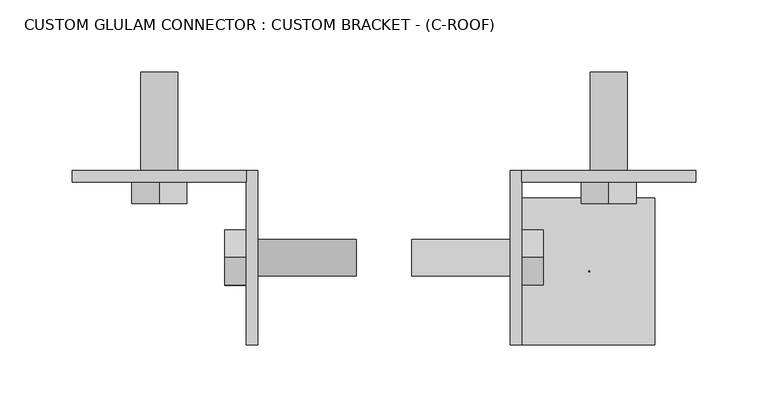
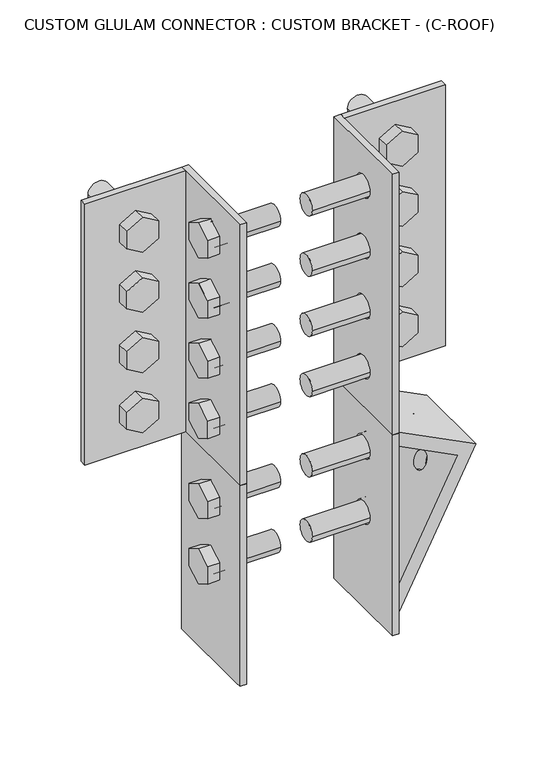
"""IFC4 building model written with IfcOpenShell, lengths in millimetres: fastener geometry, CUSTOM GLULAM CONNECTOR : CUSTOM BRACKET - (C-ROOF)."""

from ifc_helpers import new_model, si_unit, point, frame, frame_2d, origin, place, context, project, spatial, polyline, circle_curve, trimmed, segment, composite_curve, outline, extrude, source, transform, mapped, element, save
from ifc_brep_helpers import plane_surface, revolved_surface, advanced_brep


def custom_glulam_connector_custom_bracket_c_roof_f3df198d(model_context):
    return source(origin(), model_context, "Body", "SolidModel", [
        advanced_brep(
        [(-95.25, 60.325, 7.9375), (-95.25, 60.325, 261.9375), (-87.3125, 60.325, 261.9375), (-87.3125, 60.325, 7.9375), (-95.25, -60.325, 261.9375), (-95.25, -60.325, 7.9375), (-87.3125, -60.325, 7.9375), (-87.3125, -60.325, 261.9375), (-95.25, 13.890625, 128.5875), (-87.3125, 13.890625, 128.5875), (-87.3125, -13.890625, 128.5875), (-95.25, -13.890625, 128.5875), (-95.25, -52.3875, 261.9375), (-95.25, -52.3875, 7.9375), (-95.25, -13.890625, 211.1375), (-95.25, 13.890625, 211.1375), (-87.3125, 13.890625, 211.1375), (-87.3125, -13.890625, 211.1375)],
        [
            (0, 1),
            (1, 2),
            (2, 3),
            (3, 0),
            (4, 5),
            (5, 6),
            (6, 7),
            (7, 4),
            (8, 9),
            (9, 10, circle_curve(frame((-87.3125, 0.0, 128.5875), z_axis=(1.0, 0.0, 0.0), x_axis=(0.0, -1.0, 0.0)), 13.890625)),
            (10, 11),
            (11, 8, circle_curve(frame((-95.25, 0.0, 128.5875), z_axis=(-1.0, 0.0, 0.0), x_axis=(0.0, -1.0, 0.0)), 13.890625)),
            (4, 12),
            (12, 1),
            (0, 13),
            (13, 5),
            (11, 8, circle_curve(frame((-95.25, 0.0, 128.5875), z_axis=(1.0, 0.0, 0.0), x_axis=(0.0, -1.0, 0.0)), 13.890625)),
            (14, 15, circle_curve(frame((-95.25, 0.0, 211.1375), z_axis=(1.0, 0.0, 0.0), x_axis=(0.0, -1.0, 0.0)), 13.890625)),
            (15, 14, circle_curve(frame((-95.25, 0.0, 211.1375), z_axis=(1.0, 0.0, 0.0), x_axis=(0.0, -1.0, 0.0)), 13.890625)),
            (16, 15),
            (14, 17),
            (17, 16, circle_curve(frame((-87.3125, 0.0, 211.1375), z_axis=(1.0, 0.0, 0.0), x_axis=(0.0, -1.0, 0.0)), 13.890625)),
            (16, 17, circle_curve(frame((-87.3125, 0.0, 211.1375), z_axis=(1.0, 0.0, 0.0), x_axis=(0.0, -1.0, 0.0)), 13.890625)),
            (10, 9, circle_curve(frame((-87.3125, 0.0, 128.5875), z_axis=(1.0, 0.0, 0.0), x_axis=(0.0, -1.0, 0.0)), 13.890625)),
            (6, 3),
            (2, 7),
        ],
        [
            plane_surface(frame((-95.25, 60.325, 261.9375), z_axis=(0.0, 1.0, 0.0), x_axis=(1.0, 0.0, 0.0))),
            plane_surface(frame((-95.25, -60.325, 7.9375), z_axis=(0.0, -1.0, 0.0), x_axis=(1.0, 0.0, 0.0))),
            revolved_surface(polyline([(-95.25, -13.890625, 128.5875), (-87.3125, -13.890625, 128.5875)]), (-87.3125, 0.0, 128.5875), (-1.0, 0.0, 0.0)),
            plane_surface(frame((-95.25, 60.325, 261.9375), z_axis=(-1.0, 0.0, 0.0), x_axis=(0.0, 1.0, 0.0))),
            revolved_surface(polyline([(-95.25, -13.890625, 211.1375), (-87.3125, -13.890625, 211.1375)]), (-87.3125, 0.0, 211.1375), (-1.0, 0.0, 0.0)),
            plane_surface(frame((-87.3125, 60.325, 261.9375), z_axis=(1.0, 0.0, 0.0), x_axis=(0.0, -1.0, 0.0))),
            plane_surface(frame((-95.25, -60.325, 261.9375), z_axis=(0.0, 0.0, 1.0), x_axis=(1.0, 0.0, 0.0))),
            plane_surface(frame((-95.25, 60.325, 7.9375), z_axis=(0.0, 0.0, -1.0), x_axis=(1.0, 0.0, 0.0))),
        ],
        [
            (0, [[1, 2, 3, 4]]),
            (1, [[5, 6, 7, 8]]),
            (2, [[9, 10, 11, 12]]),
            (3, [[13, 14, -1, 15, 16, -5], [17, -12], [18, 19]]),
            (4, [[20, -18, 21, 22]]),
            (4, [[-20, 23, -21, -19]]),
            (2, [[-9, -17, -11, 24]]),
            (5, [[-7, 25, -3, 26], [-22, -23], [-24, -10]]),
            (6, [[-14, -13, -8, -26, -2]]),
            (7, [[-16, -15, -4, -25, -6]]),
        ],
    ),
        extrude(outline(polyline([(19.05, 222.1360226), (19.05, 200.1389774), (0.0, 189.1404547), (-19.05, 200.1389774), (-19.05, 222.1360226), (0.0, 233.1345453), (19.05, 222.1360226)])), frame((-110.2320312, 0.0, 0.0), z_axis=(1.0, 0.0, 0.0), x_axis=(0.0, 1.0, 0.0)), (0.0, 0.0, 1.0), 14.9820312),
        extrude(outline(composite_curve([segment(trimmed(circle_curve(frame_2d((0.0, 211.1375)), 12.7), [point((12.7, 211.1375))], [point((-12.7, 211.1375))], False, "CARTESIAN"), True, "CONTINUOUS"), segment(trimmed(circle_curve(frame_2d((0.0, 211.1375)), 12.7), [point((-12.7, 211.1375))], [point((12.7, 211.1375))], False, "CARTESIAN"), True, "CONTINUOUS")], self_intersect=False)), frame((-95.25, 0.0, 0.0), z_axis=(1.0, 0.0, 0.0), x_axis=(0.0, 1.0, 0.0)), (0.0, 0.0, 1.0), 76.2),
        extrude(outline(polyline([(19.05, 139.5860226), (19.05, 117.5889774), (0.0, 106.5904547), (-19.05, 117.5889774), (-19.05, 139.5860226), (0.0, 150.5845453), (19.05, 139.5860226)])), frame((-110.2320312, 0.0, 0.0), z_axis=(1.0, 0.0, 0.0), x_axis=(0.0, 1.0, 0.0)), (0.0, 0.0, 1.0), 14.9820312),
        extrude(outline(composite_curve([segment(trimmed(circle_curve(frame_2d((0.0, 128.5875)), 12.7), [point((12.7, 128.5875))], [point((-12.7, 128.5875))], False, "CARTESIAN"), True, "CONTINUOUS"), segment(trimmed(circle_curve(frame_2d((0.0, 128.5875)), 12.7), [point((-12.7, 128.5875))], [point((12.7, 128.5875))], False, "CARTESIAN"), True, "CONTINUOUS")], self_intersect=False)), frame((-95.25, 0.0, 0.0), z_axis=(1.0, 0.0, 0.0), x_axis=(0.0, 1.0, 0.0)), (0.0, 0.0, 1.0), 76.2),
        extrude(outline(polyline([(19.05, 222.1360226), (19.05, 200.1389774), (0.0, 189.1404547), (-19.05, 200.1389774), (-19.05, 222.1360226), (0.0, 233.1345453), (19.05, 222.1360226)])), frame((-110.2320312, 0.0, 0.0), z_axis=(1.0, 0.0, 0.0), x_axis=(0.0, 1.0, 0.0)), (0.0, 0.0, 1.0), 14.9820312),
        extrude(outline(composite_curve([segment(trimmed(circle_curve(frame_2d((0.0, 211.1375)), 12.7), [point((12.7, 211.1375))], [point((-12.7, 211.1375))], False, "CARTESIAN"), True, "CONTINUOUS"), segment(trimmed(circle_curve(frame_2d((0.0, 211.1375)), 12.7), [point((-12.7, 211.1375))], [point((12.7, 211.1375))], False, "CARTESIAN"), True, "CONTINUOUS")], self_intersect=False)), frame((-95.25, 0.0, 0.0), z_axis=(1.0, 0.0, 0.0), x_axis=(0.0, 1.0, 0.0)), (0.0, 0.0, 1.0), 76.2),
        advanced_brep(
        [(95.25, 60.325, 7.9375), (87.3125, 60.325, 7.9375), (87.3125, 60.325, 261.9375), (95.25, 60.325, 261.9375), (95.25, -60.325, 261.9375), (87.3125, -60.325, 261.9375), (87.3125, -60.325, 7.9375), (95.25, -60.325, 7.9375), (95.25, 13.890625, 128.5875), (95.25, -13.890625, 128.5875), (87.3125, -13.890625, 128.5875), (87.3125, 13.890625, 128.5875), (95.25, -52.3875, 7.9375), (95.25, -52.3875, 261.9375), (95.25, -13.890625, 211.1375), (95.25, 13.890625, 211.1375), (87.3125, 13.890625, 211.1375), (87.3125, -13.890625, 211.1375)],
        [
            (0, 1),
            (1, 2),
            (2, 3),
            (3, 0),
            (4, 5),
            (5, 6),
            (6, 7),
            (7, 4),
            (8, 9, circle_curve(frame((95.25, 0.0, 128.5875), z_axis=(1.0, 0.0, 0.0), x_axis=(0.0, -1.0, 0.0)), 13.890625)),
            (9, 10),
            (10, 11, circle_curve(frame((87.3125, 0.0, 128.5875), z_axis=(-1.0, 0.0, 0.0), x_axis=(0.0, -1.0, 0.0)), 13.890625)),
            (11, 8),
            (7, 12),
            (12, 0),
            (3, 13),
            (13, 4),
            (14, 15, circle_curve(frame((95.25, 0.0, 211.1375), z_axis=(-1.0, 0.0, 0.0), x_axis=(0.0, -1.0, 0.0)), 13.890625)),
            (15, 14, circle_curve(frame((95.25, 0.0, 211.1375), z_axis=(-1.0, 0.0, 0.0), x_axis=(0.0, -1.0, 0.0)), 13.890625)),
            (8, 9, circle_curve(frame((95.25, 0.0, 128.5875), z_axis=(-1.0, 0.0, 0.0), x_axis=(0.0, -1.0, 0.0)), 13.890625)),
            (16, 17, circle_curve(frame((87.3125, 0.0, 211.1375), z_axis=(-1.0, 0.0, 0.0), x_axis=(0.0, -1.0, 0.0)), 13.890625)),
            (17, 14),
            (15, 16),
            (17, 16, circle_curve(frame((87.3125, 0.0, 211.1375), z_axis=(-1.0, 0.0, 0.0), x_axis=(0.0, -1.0, 0.0)), 13.890625)),
            (11, 10, circle_curve(frame((87.3125, 0.0, 128.5875), z_axis=(-1.0, 0.0, 0.0), x_axis=(0.0, -1.0, 0.0)), 13.890625)),
            (5, 2),
            (1, 6),
        ],
        [
            plane_surface(frame((95.25, 60.325, 261.9375), z_axis=(0.0, 1.0, 0.0), x_axis=(-1.0, 0.0, 0.0))),
            plane_surface(frame((95.25, -60.325, 7.9375), z_axis=(0.0, -1.0, 0.0), x_axis=(-1.0, 0.0, 0.0))),
            revolved_surface(polyline([(95.25, -13.890625, 128.5875), (87.3125, -13.890625, 128.5875)]), (87.3125, 0.0, 128.5875), (1.0, 0.0, 0.0)),
            plane_surface(frame((95.25, 60.325, 261.9375), z_axis=(1.0, 0.0, 0.0), x_axis=(0.0, 1.0, 0.0))),
            revolved_surface(polyline([(95.25, -13.890625, 211.1375), (87.3125, -13.890625, 211.1375)]), (87.3125, 0.0, 211.1375), (1.0, 0.0, 0.0)),
            plane_surface(frame((87.3125, 60.325, 261.9375), z_axis=(-1.0, 0.0, 0.0), x_axis=(0.0, -1.0, 0.0))),
            plane_surface(frame((95.25, -60.325, 261.9375), z_axis=(0.0, 0.0, 1.0), x_axis=(-1.0, 0.0, 0.0))),
            plane_surface(frame((95.25, 60.325, 7.9375), z_axis=(0.0, 0.0, -1.0), x_axis=(-1.0, 0.0, 0.0))),
        ],
        [
            (0, [[1, 2, 3, 4]]),
            (1, [[5, 6, 7, 8]]),
            (2, [[9, 10, 11, 12]]),
            (3, [[-8, 13, 14, -4, 15, 16], [17, 18], [-9, 19]]),
            (4, [[20, 21, -18, 22]]),
            (4, [[-17, -21, 23, -22]]),
            (2, [[24, -10, -19, -12]]),
            (5, [[25, -2, 26, -6], [-23, -20], [-11, -24]]),
            (6, [[-3, -25, -5, -16, -15]]),
            (7, [[-7, -26, -1, -14, -13]]),
        ],
    ),
        extrude(outline(polyline([(19.05, 222.1360226), (19.05, 200.1389774), (0.0, 189.1404547), (-19.05, 200.1389774), (-19.05, 222.1360226), (0.0, 233.1345453), (19.05, 222.1360226)])), frame((95.25, 0.0, 0.0), z_axis=(1.0, 0.0, 0.0), x_axis=(0.0, 1.0, 0.0)), (0.0, 0.0, 1.0), 14.9820312),
        extrude(outline(composite_curve([segment(trimmed(circle_curve(frame_2d((0.0, 211.1375)), 12.7), [point((12.7, 211.1375))], [point((-12.7, 211.1375))], False, "CARTESIAN"), True, "CONTINUOUS"), segment(trimmed(circle_curve(frame_2d((0.0, 211.1375)), 12.7), [point((-12.7, 211.1375))], [point((12.7, 211.1375))], False, "CARTESIAN"), True, "CONTINUOUS")], self_intersect=False)), frame((19.05, 0.0, 0.0), z_axis=(1.0, 0.0, 0.0), x_axis=(0.0, 1.0, 0.0)), (0.0, 0.0, 1.0), 76.2),
        extrude(outline(polyline([(19.05, 139.5860226), (19.05, 117.5889774), (0.0, 106.5904547), (-19.05, 117.5889774), (-19.05, 139.5860226), (0.0, 150.5845453), (19.05, 139.5860226)])), frame((95.25, 0.0, 0.0), z_axis=(1.0, 0.0, 0.0), x_axis=(0.0, 1.0, 0.0)), (0.0, 0.0, 1.0), 14.9820312),
        extrude(outline(composite_curve([segment(trimmed(circle_curve(frame_2d((0.0, 128.5875)), 12.7), [point((12.7, 128.5875))], [point((-12.7, 128.5875))], False, "CARTESIAN"), True, "CONTINUOUS"), segment(trimmed(circle_curve(frame_2d((0.0, 128.5875)), 12.7), [point((-12.7, 128.5875))], [point((12.7, 128.5875))], False, "CARTESIAN"), True, "CONTINUOUS")], self_intersect=False)), frame((19.05, 0.0, 0.0), z_axis=(1.0, 0.0, 0.0), x_axis=(0.0, 1.0, 0.0)), (0.0, 0.0, 1.0), 76.2),
        extrude(outline(polyline([(19.05, 222.1360226), (19.05, 200.1389774), (0.0, 189.1404547), (-19.05, 200.1389774), (-19.05, 222.1360226), (0.0, 233.1345453), (19.05, 222.1360226)])), frame((95.25, 0.0, 0.0), z_axis=(1.0, 0.0, 0.0), x_axis=(0.0, 1.0, 0.0)), (0.0, 0.0, 1.0), 14.9820312),
        extrude(outline(composite_curve([segment(trimmed(circle_curve(frame_2d((0.0, 211.1375)), 12.7), [point((12.7, 211.1375))], [point((-12.7, 211.1375))], False, "CARTESIAN"), True, "CONTINUOUS"), segment(trimmed(circle_curve(frame_2d((0.0, 211.1375)), 12.7), [point((-12.7, 211.1375))], [point((12.7, 211.1375))], False, "CARTESIAN"), True, "CONTINUOUS")], self_intersect=False)), frame((19.05, 0.0, 0.0), z_axis=(1.0, 0.0, 0.0), x_axis=(0.0, 1.0, 0.0)), (0.0, 0.0, 1.0), 76.2),
        extrude(outline(polyline([(592.1375, -215.9), (261.9375, -215.9), (261.9375, -95.25), (592.1375, -95.25), (592.1375, -215.9)]), holes=[composite_curve([segment(trimmed(circle_curve(frame_2d((465.1375, -155.575)), 13.890625), [point((465.1375, -169.465625))], [point((465.1375, -141.684375))], True, "CARTESIAN"), True, "CONTINUOUS"), segment(trimmed(circle_curve(frame_2d((465.1375, -155.575)), 13.890625), [point((465.1375, -141.684375))], [point((465.1375, -169.465625))], True, "CARTESIAN"), True, "CONTINUOUS")], self_intersect=False), composite_curve([segment(trimmed(circle_curve(frame_2d((388.9375, -155.575)), 13.890625), [point((388.9375, -169.465625))], [point((388.9375, -141.684375))], True, "CARTESIAN"), True, "CONTINUOUS"), segment(trimmed(circle_curve(frame_2d((388.9375, -155.575)), 13.890625), [point((388.9375, -141.684375))], [point((388.9375, -169.465625))], True, "CARTESIAN"), True, "CONTINUOUS")], self_intersect=False), composite_curve([segment(trimmed(circle_curve(frame_2d((312.7375, -155.575)), 13.890625), [point((312.7375, -169.465625))], [point((312.7375, -141.684375))], True, "CARTESIAN"), True, "CONTINUOUS"), segment(trimmed(circle_curve(frame_2d((312.7375, -155.575)), 13.890625), [point((312.7375, -141.684375))], [point((312.7375, -169.465625))], True, "CARTESIAN"), True, "CONTINUOUS")], self_intersect=False), composite_curve([segment(trimmed(circle_curve(frame_2d((541.3375, -155.575)), 13.890625), [point((541.3375, -169.465625))], [point((541.3375, -141.684375))], True, "CARTESIAN"), True, "CONTINUOUS"), segment(trimmed(circle_curve(frame_2d((541.3375, -155.575)), 13.890625), [point((541.3375, -141.684375))], [point((541.3375, -169.465625))], True, "CARTESIAN"), True, "CONTINUOUS")], self_intersect=False)]), frame((0.0, 52.3875, 0.0), z_axis=(0.0, 1.0, 0.0), x_axis=(0.0, 0.0, 1.0)), (0.0, 0.0, 1.0), 7.9375),
        extrude(outline(polyline([(552.3360226, -136.525), (563.3345453, -155.575), (552.3360226, -174.625), (530.3389774, -174.625), (519.3404547, -155.575), (530.3389774, -136.525), (552.3360226, -136.525)])), frame((0.0, 37.4054688, 0.0), z_axis=(0.0, 1.0, 0.0), x_axis=(0.0, 0.0, 1.0)), (0.0, 0.0, 1.0), 14.9820312),
        extrude(outline(composite_curve([segment(trimmed(circle_curve(frame_2d((541.3375, -155.575)), 12.7), [point((541.3375, -142.875))], [point((541.3375, -168.275))], False, "CARTESIAN"), True, "CONTINUOUS"), segment(trimmed(circle_curve(frame_2d((541.3375, -155.575)), 12.7), [point((541.3375, -168.275))], [point((541.3375, -142.875))], False, "CARTESIAN"), True, "CONTINUOUS")], self_intersect=False)), frame((0.0, 52.3875, 0.0), z_axis=(0.0, 1.0, 0.0), x_axis=(0.0, 0.0, 1.0)), (0.0, 0.0, 1.0), 76.2),
        extrude(outline(polyline([(476.1360226, -136.525), (487.1345453, -155.575), (476.1360226, -174.625), (454.1389774, -174.625), (443.1404547, -155.575), (454.1389774, -136.525), (476.1360226, -136.525)])), frame((0.0, 37.4054688, 0.0), z_axis=(0.0, 1.0, 0.0), x_axis=(0.0, 0.0, 1.0)), (0.0, 0.0, 1.0), 14.9820312),
        extrude(outline(composite_curve([segment(trimmed(circle_curve(frame_2d((465.1375, -155.575)), 12.7), [point((465.1375, -142.875))], [point((465.1375, -168.275))], False, "CARTESIAN"), True, "CONTINUOUS"), segment(trimmed(circle_curve(frame_2d((465.1375, -155.575)), 12.7), [point((465.1375, -168.275))], [point((465.1375, -142.875))], False, "CARTESIAN"), True, "CONTINUOUS")], self_intersect=False)), frame((0.0, 52.3875, 0.0), z_axis=(0.0, 1.0, 0.0), x_axis=(0.0, 0.0, 1.0)), (0.0, 0.0, 1.0), 76.2),
        extrude(outline(polyline([(552.3360226, -136.525), (563.3345453, -155.575), (552.3360226, -174.625), (530.3389774, -174.625), (519.3404547, -155.575), (530.3389774, -136.525), (552.3360226, -136.525)])), frame((0.0, 37.4054688, 0.0), z_axis=(0.0, 1.0, 0.0), x_axis=(0.0, 0.0, 1.0)), (0.0, 0.0, 1.0), 14.9820312),
        extrude(outline(composite_curve([segment(trimmed(circle_curve(frame_2d((541.3375, -155.575)), 12.7), [point((541.3375, -142.875))], [point((541.3375, -168.275))], False, "CARTESIAN"), True, "CONTINUOUS"), segment(trimmed(circle_curve(frame_2d((541.3375, -155.575)), 12.7), [point((541.3375, -168.275))], [point((541.3375, -142.875))], False, "CARTESIAN"), True, "CONTINUOUS")], self_intersect=False)), frame((0.0, 52.3875, 0.0), z_axis=(0.0, 1.0, 0.0), x_axis=(0.0, 0.0, 1.0)), (0.0, 0.0, 1.0), 76.2),
        extrude(outline(polyline([(399.9360226, -136.525), (410.9345453, -155.575), (399.9360226, -174.625), (377.9389774, -174.625), (366.9404547, -155.575), (377.9389774, -136.525), (399.9360226, -136.525)])), frame((0.0, 37.4054688, 0.0), z_axis=(0.0, 1.0, 0.0), x_axis=(0.0, 0.0, 1.0)), (0.0, 0.0, 1.0), 14.9820312),
        extrude(outline(composite_curve([segment(trimmed(circle_curve(frame_2d((388.9375, -155.575)), 12.7), [point((388.9375, -142.875))], [point((388.9375, -168.275))], False, "CARTESIAN"), True, "CONTINUOUS"), segment(trimmed(circle_curve(frame_2d((388.9375, -155.575)), 12.7), [point((388.9375, -168.275))], [point((388.9375, -142.875))], False, "CARTESIAN"), True, "CONTINUOUS")], self_intersect=False)), frame((0.0, 52.3875, 0.0), z_axis=(0.0, 1.0, 0.0), x_axis=(0.0, 0.0, 1.0)), (0.0, 0.0, 1.0), 76.2),
        extrude(outline(polyline([(323.7360226, -136.525), (334.7345453, -155.575), (323.7360226, -174.625), (301.7389774, -174.625), (290.7404547, -155.575), (301.7389774, -136.525), (323.7360226, -136.525)])), frame((0.0, 37.4054688, 0.0), z_axis=(0.0, 1.0, 0.0), x_axis=(0.0, 0.0, 1.0)), (0.0, 0.0, 1.0), 14.9820312),
        extrude(outline(composite_curve([segment(trimmed(circle_curve(frame_2d((312.7375, -155.575)), 12.7), [point((312.7375, -142.875))], [point((312.7375, -168.275))], False, "CARTESIAN"), True, "CONTINUOUS"), segment(trimmed(circle_curve(frame_2d((312.7375, -155.575)), 12.7), [point((312.7375, -168.275))], [point((312.7375, -142.875))], False, "CARTESIAN"), True, "CONTINUOUS")], self_intersect=False)), frame((0.0, 52.3875, 0.0), z_axis=(0.0, 1.0, 0.0), x_axis=(0.0, 0.0, 1.0)), (0.0, 0.0, 1.0), 76.2),
        advanced_brep(
        [(-95.25, 60.325, 261.9375), (-95.25, 60.325, 592.1375), (-87.3125, 60.325, 592.1375), (-87.3125, 60.325, 261.9375), (-95.25, -60.325, 592.1375), (-95.25, -60.325, 261.9375), (-87.3125, -60.325, 261.9375), (-87.3125, -60.325, 592.1375), (-95.25, 13.890625, 465.1375), (-87.3125, 13.890625, 465.1375), (-87.3125, -13.890625, 465.1375), (-95.25, -13.890625, 465.1375), (-95.25, 52.3875, 592.1375), (-95.25, 52.3875, 261.9375), (-95.25, -13.890625, 541.3375), (-95.25, 13.890625, 541.3375), (-95.25, -13.890625, 388.9375), (-95.25, 13.890625, 388.9375), (-95.25, -13.890625, 312.7375), (-95.25, 13.890625, 312.7375), (-87.3125, 13.890625, 541.3375), (-87.3125, -13.890625, 541.3375), (-87.3125, 13.890625, 388.9375), (-87.3125, -13.890625, 388.9375), (-87.3125, 13.890625, 312.7375), (-87.3125, -13.890625, 312.7375)],
        [
            (0, 1),
            (1, 2),
            (2, 3),
            (3, 0),
            (4, 5),
            (5, 6),
            (6, 7),
            (7, 4),
            (8, 9),
            (9, 10, circle_curve(frame((-87.3125, 0.0, 465.1375), z_axis=(1.0, 0.0, 0.0), x_axis=(0.0, -1.0, 0.0)), 13.890625)),
            (10, 11),
            (11, 8, circle_curve(frame((-95.25, 0.0, 465.1375), z_axis=(-1.0, 0.0, 0.0), x_axis=(0.0, -1.0, 0.0)), 13.890625)),
            (4, 12),
            (12, 1),
            (0, 13),
            (13, 5),
            (11, 8, circle_curve(frame((-95.25, 0.0, 465.1375), z_axis=(1.0, 0.0, 0.0), x_axis=(0.0, -1.0, 0.0)), 13.890625)),
            (14, 15, circle_curve(frame((-95.25, 0.0, 541.3375), z_axis=(1.0, 0.0, 0.0), x_axis=(0.0, -1.0, 0.0)), 13.890625)),
            (15, 14, circle_curve(frame((-95.25, 0.0, 541.3375), z_axis=(1.0, 0.0, 0.0), x_axis=(0.0, -1.0, 0.0)), 13.890625)),
            (16, 17, circle_curve(frame((-95.25, 0.0, 388.9375), z_axis=(1.0, 0.0, 0.0), x_axis=(0.0, -1.0, 0.0)), 13.890625)),
            (17, 16, circle_curve(frame((-95.25, 0.0, 388.9375), z_axis=(1.0, 0.0, 0.0), x_axis=(0.0, -1.0, 0.0)), 13.890625)),
            (18, 19, circle_curve(frame((-95.25, 0.0, 312.7375), z_axis=(1.0, 0.0, 0.0), x_axis=(0.0, -1.0, 0.0)), 13.890625)),
            (19, 18, circle_curve(frame((-95.25, 0.0, 312.7375), z_axis=(1.0, 0.0, 0.0), x_axis=(0.0, -1.0, 0.0)), 13.890625)),
            (20, 15),
            (14, 21),
            (21, 20, circle_curve(frame((-87.3125, 0.0, 541.3375), z_axis=(1.0, 0.0, 0.0), x_axis=(0.0, -1.0, 0.0)), 13.890625)),
            (20, 21, circle_curve(frame((-87.3125, 0.0, 541.3375), z_axis=(1.0, 0.0, 0.0), x_axis=(0.0, -1.0, 0.0)), 13.890625)),
            (10, 9, circle_curve(frame((-87.3125, 0.0, 465.1375), z_axis=(1.0, 0.0, 0.0), x_axis=(0.0, -1.0, 0.0)), 13.890625)),
            (6, 3),
            (2, 7),
            (22, 23, circle_curve(frame((-87.3125, 0.0, 388.9375), z_axis=(-1.0, 0.0, 0.0), x_axis=(0.0, -1.0, 0.0)), 13.890625)),
            (23, 22, circle_curve(frame((-87.3125, 0.0, 388.9375), z_axis=(-1.0, 0.0, 0.0), x_axis=(0.0, -1.0, 0.0)), 13.890625)),
            (24, 25, circle_curve(frame((-87.3125, 0.0, 312.7375), z_axis=(-1.0, 0.0, 0.0), x_axis=(0.0, -1.0, 0.0)), 13.890625)),
            (25, 24, circle_curve(frame((-87.3125, 0.0, 312.7375), z_axis=(-1.0, 0.0, 0.0), x_axis=(0.0, -1.0, 0.0)), 13.890625)),
            (19, 24),
            (25, 18),
            (17, 22),
            (23, 16),
        ],
        [
            plane_surface(frame((-95.25, 60.325, 592.1375), z_axis=(0.0, 1.0, 0.0), x_axis=(1.0, 0.0, 0.0))),
            plane_surface(frame((-95.25, -60.325, 261.9375), z_axis=(0.0, -1.0, 0.0), x_axis=(1.0, 0.0, 0.0))),
            revolved_surface(polyline([(-95.25, -13.890625, 465.1375), (-87.3125, -13.890625, 465.1375)]), (-87.3125, 0.0, 465.1375), (-1.0, 0.0, 0.0)),
            plane_surface(frame((-95.25, 60.325, 592.1375), z_axis=(-1.0, 0.0, 0.0), x_axis=(0.0, 1.0, 0.0))),
            revolved_surface(polyline([(-95.25, -13.890625, 541.3375), (-87.3125, -13.890625, 541.3375)]), (-87.3125, 0.0, 541.3375), (-1.0, 0.0, 0.0)),
            plane_surface(frame((-87.3125, 60.325, 592.1375), z_axis=(1.0, 0.0, 0.0), x_axis=(0.0, -1.0, 0.0))),
            plane_surface(frame((-95.25, -60.325, 592.1375), z_axis=(0.0, 0.0, 1.0), x_axis=(1.0, 0.0, 0.0))),
            plane_surface(frame((-95.25, 60.325, 261.9375), z_axis=(0.0, 0.0, -1.0), x_axis=(1.0, 0.0, 0.0))),
            revolved_surface(polyline([(-95.25, -13.890625, 312.7375), (-87.3125, -13.890625, 312.7375)]), (-87.3125, 0.0, 312.7375), (-1.0, 0.0, 0.0)),
            revolved_surface(polyline([(-95.25, -13.890625, 388.9375), (-87.3125, -13.890625, 388.9375)]), (-87.3125, 0.0, 388.9375), (-1.0, 0.0, 0.0)),
        ],
        [
            (0, [[1, 2, 3, 4]]),
            (1, [[5, 6, 7, 8]]),
            (2, [[9, 10, 11, 12]]),
            (3, [[13, 14, -1, 15, 16, -5], [17, -12], [18, 19], [20, 21], [22, 23]]),
            (4, [[24, -18, 25, 26]]),
            (4, [[-24, 27, -25, -19]]),
            (2, [[-9, -17, -11, 28]]),
            (5, [[-7, 29, -3, 30], [-26, -27], [-28, -10], [31, 32], [33, 34]]),
            (6, [[-14, -13, -8, -30, -2]]),
            (7, [[-16, -15, -4, -29, -6]]),
            (8, [[35, -34, 36, -23]]),
            (9, [[37, -32, 38, -21]]),
            (8, [[-35, -22, -36, -33]]),
            (9, [[-37, -20, -38, -31]]),
        ],
    ),
        extrude(outline(polyline([(19.05, 552.3360226), (19.05, 530.3389774), (0.0, 519.3404547), (-19.05, 530.3389774), (-19.05, 552.3360226), (0.0, 563.3345453), (19.05, 552.3360226)])), frame((-110.2320312, 0.0, 0.0), z_axis=(1.0, 0.0, 0.0), x_axis=(0.0, 1.0, 0.0)), (0.0, 0.0, 1.0), 14.9820312),
        extrude(outline(composite_curve([segment(trimmed(circle_curve(frame_2d((0.0, 541.3375)), 12.7), [point((12.7, 541.3375))], [point((-12.7, 541.3375))], False, "CARTESIAN"), True, "CONTINUOUS"), segment(trimmed(circle_curve(frame_2d((0.0, 541.3375)), 12.7), [point((-12.7, 541.3375))], [point((12.7, 541.3375))], False, "CARTESIAN"), True, "CONTINUOUS")], self_intersect=False)), frame((-95.25, 0.0, 0.0), z_axis=(1.0, 0.0, 0.0), x_axis=(0.0, 1.0, 0.0)), (0.0, 0.0, 1.0), 76.2),
        extrude(outline(polyline([(19.05, 476.1360226), (19.05, 454.1389774), (0.0, 443.1404547), (-19.05, 454.1389774), (-19.05, 476.1360226), (0.0, 487.1345453), (19.05, 476.1360226)])), frame((-110.2320312, 0.0, 0.0), z_axis=(1.0, 0.0, 0.0), x_axis=(0.0, 1.0, 0.0)), (0.0, 0.0, 1.0), 14.9820312),
        extrude(outline(composite_curve([segment(trimmed(circle_curve(frame_2d((0.0, 465.1375)), 12.7), [point((12.7, 465.1375))], [point((-12.7, 465.1375))], False, "CARTESIAN"), True, "CONTINUOUS"), segment(trimmed(circle_curve(frame_2d((0.0, 465.1375)), 12.7), [point((-12.7, 465.1375))], [point((12.7, 465.1375))], False, "CARTESIAN"), True, "CONTINUOUS")], self_intersect=False)), frame((-95.25, 0.0, 0.0), z_axis=(1.0, 0.0, 0.0), x_axis=(0.0, 1.0, 0.0)), (0.0, 0.0, 1.0), 76.2),
        extrude(outline(polyline([(19.05, 552.3360226), (19.05, 530.3389774), (0.0, 519.3404547), (-19.05, 530.3389774), (-19.05, 552.3360226), (0.0, 563.3345453), (19.05, 552.3360226)])), frame((-110.2320312, 0.0, 0.0), z_axis=(1.0, 0.0, 0.0), x_axis=(0.0, 1.0, 0.0)), (0.0, 0.0, 1.0), 14.9820312),
        extrude(outline(composite_curve([segment(trimmed(circle_curve(frame_2d((0.0, 541.3375)), 12.7), [point((12.7, 541.3375))], [point((-12.7, 541.3375))], False, "CARTESIAN"), True, "CONTINUOUS"), segment(trimmed(circle_curve(frame_2d((0.0, 541.3375)), 12.7), [point((-12.7, 541.3375))], [point((12.7, 541.3375))], False, "CARTESIAN"), True, "CONTINUOUS")], self_intersect=False)), frame((-95.25, 0.0, 0.0), z_axis=(1.0, 0.0, 0.0), x_axis=(0.0, 1.0, 0.0)), (0.0, 0.0, 1.0), 76.2),
        extrude(outline(polyline([(19.05, 399.9360226), (19.05, 377.9389774), (0.0, 366.9404547), (-19.05, 377.9389774), (-19.05, 399.9360226), (0.0, 410.9345453), (19.05, 399.9360226)])), frame((-110.2320312, 0.0, 0.0), z_axis=(1.0, 0.0, 0.0), x_axis=(0.0, 1.0, 0.0)), (0.0, 0.0, 1.0), 14.9820312),
        extrude(outline(composite_curve([segment(trimmed(circle_curve(frame_2d((0.0, 388.9375)), 12.7), [point((12.7, 388.9375))], [point((-12.7, 388.9375))], False, "CARTESIAN"), True, "CONTINUOUS"), segment(trimmed(circle_curve(frame_2d((0.0, 388.9375)), 12.7), [point((-12.7, 388.9375))], [point((12.7, 388.9375))], False, "CARTESIAN"), True, "CONTINUOUS")], self_intersect=False)), frame((-95.25, 0.0, 0.0), z_axis=(1.0, 0.0, 0.0), x_axis=(0.0, 1.0, 0.0)), (0.0, 0.0, 1.0), 76.2),
        extrude(outline(polyline([(19.05, 323.7360226), (19.05, 301.7389774), (0.0, 290.7404547), (-19.05, 301.7389774), (-19.05, 323.7360226), (0.0, 334.7345453), (19.05, 323.7360226)])), frame((-110.2320312, 0.0, 0.0), z_axis=(1.0, 0.0, 0.0), x_axis=(0.0, 1.0, 0.0)), (0.0, 0.0, 1.0), 14.9820312),
        extrude(outline(composite_curve([segment(trimmed(circle_curve(frame_2d((0.0, 312.7375)), 12.7), [point((12.7, 312.7375))], [point((-12.7, 312.7375))], False, "CARTESIAN"), True, "CONTINUOUS"), segment(trimmed(circle_curve(frame_2d((0.0, 312.7375)), 12.7), [point((-12.7, 312.7375))], [point((12.7, 312.7375))], False, "CARTESIAN"), True, "CONTINUOUS")], self_intersect=False)), frame((-95.25, 0.0, 0.0), z_axis=(1.0, 0.0, 0.0), x_axis=(0.0, 1.0, 0.0)), (0.0, 0.0, 1.0), 76.2),
        extrude(outline(polyline([(592.1375, 215.9), (592.1375, 95.25), (261.9375, 95.25), (261.9375, 215.9), (592.1375, 215.9)]), holes=[composite_curve([segment(trimmed(circle_curve(frame_2d((465.1375, 155.575)), 13.890625), [point((465.1375, 169.465625))], [point((465.1375, 141.684375))], True, "CARTESIAN"), True, "CONTINUOUS"), segment(trimmed(circle_curve(frame_2d((465.1375, 155.575)), 13.890625), [point((465.1375, 141.684375))], [point((465.1375, 169.465625))], True, "CARTESIAN"), True, "CONTINUOUS")], self_intersect=False), composite_curve([segment(trimmed(circle_curve(frame_2d((388.9375, 155.575)), 13.890625), [point((388.9375, 169.465625))], [point((388.9375, 141.684375))], True, "CARTESIAN"), True, "CONTINUOUS"), segment(trimmed(circle_curve(frame_2d((388.9375, 155.575)), 13.890625), [point((388.9375, 141.684375))], [point((388.9375, 169.465625))], True, "CARTESIAN"), True, "CONTINUOUS")], self_intersect=False), composite_curve([segment(trimmed(circle_curve(frame_2d((541.3375, 155.575)), 13.890625), [point((541.3375, 169.465625))], [point((541.3375, 141.684375))], True, "CARTESIAN"), True, "CONTINUOUS"), segment(trimmed(circle_curve(frame_2d((541.3375, 155.575)), 13.890625), [point((541.3375, 141.684375))], [point((541.3375, 169.465625))], True, "CARTESIAN"), True, "CONTINUOUS")], self_intersect=False), composite_curve([segment(trimmed(circle_curve(frame_2d((312.7375, 155.575)), 13.890625), [point((312.7375, 169.465625))], [point((312.7375, 141.684375))], True, "CARTESIAN"), True, "CONTINUOUS"), segment(trimmed(circle_curve(frame_2d((312.7375, 155.575)), 13.890625), [point((312.7375, 141.684375))], [point((312.7375, 169.465625))], True, "CARTESIAN"), True, "CONTINUOUS")], self_intersect=False)]), frame((0.0, 52.3875, 0.0), z_axis=(0.0, 1.0, 0.0), x_axis=(0.0, 0.0, 1.0)), (0.0, 0.0, 1.0), 7.9375),
        extrude(outline(polyline([(552.3360226, 136.525), (530.3389774, 136.525), (519.3404547, 155.575), (530.3389774, 174.625), (552.3360226, 174.625), (563.3345453, 155.575), (552.3360226, 136.525)])), frame((0.0, 37.4054688, 0.0), z_axis=(0.0, 1.0, 0.0), x_axis=(0.0, 0.0, 1.0)), (0.0, 0.0, 1.0), 14.9820312),
        extrude(outline(composite_curve([segment(trimmed(circle_curve(frame_2d((541.3375, 155.575)), 12.7), [point((541.3375, 142.875))], [point((541.3375, 168.275))], False, "CARTESIAN"), True, "CONTINUOUS"), segment(trimmed(circle_curve(frame_2d((541.3375, 155.575)), 12.7), [point((541.3375, 168.275))], [point((541.3375, 142.875))], False, "CARTESIAN"), True, "CONTINUOUS")], self_intersect=False)), frame((0.0, 52.3875, 0.0), z_axis=(0.0, 1.0, 0.0), x_axis=(0.0, 0.0, 1.0)), (0.0, 0.0, 1.0), 76.2),
        extrude(outline(polyline([(476.1360226, 136.525), (454.1389774, 136.525), (443.1404547, 155.575), (454.1389774, 174.625), (476.1360226, 174.625), (487.1345453, 155.575), (476.1360226, 136.525)])), frame((0.0, 37.4054688, 0.0), z_axis=(0.0, 1.0, 0.0), x_axis=(0.0, 0.0, 1.0)), (0.0, 0.0, 1.0), 14.9820312),
        extrude(outline(composite_curve([segment(trimmed(circle_curve(frame_2d((465.1375, 155.575)), 12.7), [point((465.1375, 142.875))], [point((465.1375, 168.275))], False, "CARTESIAN"), True, "CONTINUOUS"), segment(trimmed(circle_curve(frame_2d((465.1375, 155.575)), 12.7), [point((465.1375, 168.275))], [point((465.1375, 142.875))], False, "CARTESIAN"), True, "CONTINUOUS")], self_intersect=False)), frame((0.0, 52.3875, 0.0), z_axis=(0.0, 1.0, 0.0), x_axis=(0.0, 0.0, 1.0)), (0.0, 0.0, 1.0), 76.2),
        extrude(outline(polyline([(552.3360226, 136.525), (530.3389774, 136.525), (519.3404547, 155.575), (530.3389774, 174.625), (552.3360226, 174.625), (563.3345453, 155.575), (552.3360226, 136.525)])), frame((0.0, 37.4054688, 0.0), z_axis=(0.0, 1.0, 0.0), x_axis=(0.0, 0.0, 1.0)), (0.0, 0.0, 1.0), 14.9820312),
        extrude(outline(composite_curve([segment(trimmed(circle_curve(frame_2d((541.3375, 155.575)), 12.7), [point((541.3375, 142.875))], [point((541.3375, 168.275))], False, "CARTESIAN"), True, "CONTINUOUS"), segment(trimmed(circle_curve(frame_2d((541.3375, 155.575)), 12.7), [point((541.3375, 168.275))], [point((541.3375, 142.875))], False, "CARTESIAN"), True, "CONTINUOUS")], self_intersect=False)), frame((0.0, 52.3875, 0.0), z_axis=(0.0, 1.0, 0.0), x_axis=(0.0, 0.0, 1.0)), (0.0, 0.0, 1.0), 76.2),
        extrude(outline(polyline([(399.9360226, 136.525), (377.9389774, 136.525), (366.9404547, 155.575), (377.9389774, 174.625), (399.9360226, 174.625), (410.9345453, 155.575), (399.9360226, 136.525)])), frame((0.0, 37.4054688, 0.0), z_axis=(0.0, 1.0, 0.0), x_axis=(0.0, 0.0, 1.0)), (0.0, 0.0, 1.0), 14.9820312),
        extrude(outline(composite_curve([segment(trimmed(circle_curve(frame_2d((388.9375, 155.575)), 12.7), [point((388.9375, 142.875))], [point((388.9375, 168.275))], False, "CARTESIAN"), True, "CONTINUOUS"), segment(trimmed(circle_curve(frame_2d((388.9375, 155.575)), 12.7), [point((388.9375, 168.275))], [point((388.9375, 142.875))], False, "CARTESIAN"), True, "CONTINUOUS")], self_intersect=False)), frame((0.0, 52.3875, 0.0), z_axis=(0.0, 1.0, 0.0), x_axis=(0.0, 0.0, 1.0)), (0.0, 0.0, 1.0), 76.2),
        extrude(outline(polyline([(323.7360226, 136.525), (301.7389774, 136.525), (290.7404547, 155.575), (301.7389774, 174.625), (323.7360226, 174.625), (334.7345453, 155.575), (323.7360226, 136.525)])), frame((0.0, 37.4054688, 0.0), z_axis=(0.0, 1.0, 0.0), x_axis=(0.0, 0.0, 1.0)), (0.0, 0.0, 1.0), 14.9820312),
        extrude(outline(composite_curve([segment(trimmed(circle_curve(frame_2d((312.7375, 155.575)), 12.7), [point((312.7375, 142.875))], [point((312.7375, 168.275))], False, "CARTESIAN"), True, "CONTINUOUS"), segment(trimmed(circle_curve(frame_2d((312.7375, 155.575)), 12.7), [point((312.7375, 168.275))], [point((312.7375, 142.875))], False, "CARTESIAN"), True, "CONTINUOUS")], self_intersect=False)), frame((0.0, 52.3875, 0.0), z_axis=(0.0, 1.0, 0.0), x_axis=(0.0, 0.0, 1.0)), (0.0, 0.0, 1.0), 76.2),
        advanced_brep(
        [(95.25, 60.325, 261.9375), (87.3125, 60.325, 261.9375), (87.3125, 60.325, 592.1375), (95.25, 60.325, 592.1375), (95.25, -60.325, 592.1375), (87.3125, -60.325, 592.1375), (87.3125, -60.325, 261.9375), (95.25, -60.325, 261.9375), (95.25, 13.890625, 465.1375), (95.25, -13.890625, 465.1375), (87.3125, -13.890625, 465.1375), (87.3125, 13.890625, 465.1375), (95.25, 52.3875, 261.9375), (95.25, 52.3875, 592.1375), (95.25, -13.890625, 541.3375), (95.25, 13.890625, 541.3375), (95.25, -13.890625, 388.9375), (95.25, 13.890625, 388.9375), (95.25, -13.890625, 312.7375), (95.25, 13.890625, 312.7375), (87.3125, 13.890625, 541.3375), (87.3125, -13.890625, 541.3375), (87.3125, 13.890625, 388.9375), (87.3125, -13.890625, 388.9375), (87.3125, 13.890625, 312.7375), (87.3125, -13.890625, 312.7375)],
        [
            (0, 1),
            (1, 2),
            (2, 3),
            (3, 0),
            (4, 5),
            (5, 6),
            (6, 7),
            (7, 4),
            (8, 9, circle_curve(frame((95.25, 0.0, 465.1375), z_axis=(1.0, 0.0, 0.0), x_axis=(0.0, -1.0, 0.0)), 13.890625)),
            (9, 10),
            (10, 11, circle_curve(frame((87.3125, 0.0, 465.1375), z_axis=(-1.0, 0.0, 0.0), x_axis=(0.0, -1.0, 0.0)), 13.890625)),
            (11, 8),
            (7, 12),
            (12, 0),
            (3, 13),
            (13, 4),
            (14, 15, circle_curve(frame((95.25, 0.0, 541.3375), z_axis=(-1.0, 0.0, 0.0), x_axis=(0.0, -1.0, 0.0)), 13.890625)),
            (15, 14, circle_curve(frame((95.25, 0.0, 541.3375), z_axis=(-1.0, 0.0, 0.0), x_axis=(0.0, -1.0, 0.0)), 13.890625)),
            (8, 9, circle_curve(frame((95.25, 0.0, 465.1375), z_axis=(-1.0, 0.0, 0.0), x_axis=(0.0, -1.0, 0.0)), 13.890625)),
            (16, 17, circle_curve(frame((95.25, 0.0, 388.9375), z_axis=(-1.0, 0.0, 0.0), x_axis=(0.0, -1.0, 0.0)), 13.890625)),
            (17, 16, circle_curve(frame((95.25, 0.0, 388.9375), z_axis=(-1.0, 0.0, 0.0), x_axis=(0.0, -1.0, 0.0)), 13.890625)),
            (18, 19, circle_curve(frame((95.25, 0.0, 312.7375), z_axis=(-1.0, 0.0, 0.0), x_axis=(0.0, -1.0, 0.0)), 13.890625)),
            (19, 18, circle_curve(frame((95.25, 0.0, 312.7375), z_axis=(-1.0, 0.0, 0.0), x_axis=(0.0, -1.0, 0.0)), 13.890625)),
            (20, 21, circle_curve(frame((87.3125, 0.0, 541.3375), z_axis=(-1.0, 0.0, 0.0), x_axis=(0.0, -1.0, 0.0)), 13.890625)),
            (21, 14),
            (15, 20),
            (21, 20, circle_curve(frame((87.3125, 0.0, 541.3375), z_axis=(-1.0, 0.0, 0.0), x_axis=(0.0, -1.0, 0.0)), 13.890625)),
            (11, 10, circle_curve(frame((87.3125, 0.0, 465.1375), z_axis=(-1.0, 0.0, 0.0), x_axis=(0.0, -1.0, 0.0)), 13.890625)),
            (5, 2),
            (1, 6),
            (22, 23, circle_curve(frame((87.3125, 0.0, 388.9375), z_axis=(1.0, 0.0, 0.0), x_axis=(0.0, -1.0, 0.0)), 13.890625)),
            (23, 22, circle_curve(frame((87.3125, 0.0, 388.9375), z_axis=(1.0, 0.0, 0.0), x_axis=(0.0, -1.0, 0.0)), 13.890625)),
            (24, 25, circle_curve(frame((87.3125, 0.0, 312.7375), z_axis=(1.0, 0.0, 0.0), x_axis=(0.0, -1.0, 0.0)), 13.890625)),
            (25, 24, circle_curve(frame((87.3125, 0.0, 312.7375), z_axis=(1.0, 0.0, 0.0), x_axis=(0.0, -1.0, 0.0)), 13.890625)),
            (18, 25),
            (24, 19),
            (16, 23),
            (22, 17),
        ],
        [
            plane_surface(frame((95.25, 60.325, 592.1375), z_axis=(0.0, 1.0, 0.0), x_axis=(-1.0, 0.0, 0.0))),
            plane_surface(frame((95.25, -60.325, 261.9375), z_axis=(0.0, -1.0, 0.0), x_axis=(-1.0, 0.0, 0.0))),
            revolved_surface(polyline([(95.25, -13.890625, 465.1375), (87.3125, -13.890625, 465.1375)]), (87.3125, 0.0, 465.1375), (1.0, 0.0, 0.0)),
            plane_surface(frame((95.25, 60.325, 592.1375), z_axis=(1.0, 0.0, 0.0), x_axis=(0.0, 1.0, 0.0))),
            revolved_surface(polyline([(95.25, -13.890625, 541.3375), (87.3125, -13.890625, 541.3375)]), (87.3125, 0.0, 541.3375), (1.0, 0.0, 0.0)),
            plane_surface(frame((87.3125, 60.325, 592.1375), z_axis=(-1.0, 0.0, 0.0), x_axis=(0.0, -1.0, 0.0))),
            plane_surface(frame((95.25, -60.325, 592.1375), z_axis=(0.0, 0.0, 1.0), x_axis=(-1.0, 0.0, 0.0))),
            plane_surface(frame((95.25, 60.325, 261.9375), z_axis=(0.0, 0.0, -1.0), x_axis=(-1.0, 0.0, 0.0))),
            revolved_surface(polyline([(95.25, -13.890625, 312.7375), (87.3125, -13.890625, 312.7375)]), (87.3125, 0.0, 312.7375), (1.0, 0.0, 0.0)),
            revolved_surface(polyline([(95.25, -13.890625, 388.9375), (87.3125, -13.890625, 388.9375)]), (87.3125, 0.0, 388.9375), (1.0, 0.0, 0.0)),
        ],
        [
            (0, [[1, 2, 3, 4]]),
            (1, [[5, 6, 7, 8]]),
            (2, [[9, 10, 11, 12]]),
            (3, [[-8, 13, 14, -4, 15, 16], [17, 18], [-9, 19], [20, 21], [22, 23]]),
            (4, [[24, 25, -18, 26]]),
            (4, [[-17, -25, 27, -26]]),
            (2, [[28, -10, -19, -12]]),
            (5, [[29, -2, 30, -6], [-27, -24], [-11, -28], [31, 32], [33, 34]]),
            (6, [[-3, -29, -5, -16, -15]]),
            (7, [[-7, -30, -1, -14, -13]]),
            (8, [[-22, 35, -33, 36]]),
            (9, [[-20, 37, -31, 38]]),
            (8, [[-34, -35, -23, -36]]),
            (9, [[-32, -37, -21, -38]]),
        ],
    ),
        extrude(outline(polyline([(19.05, 552.3360226), (19.05, 530.3389774), (0.0, 519.3404547), (-19.05, 530.3389774), (-19.05, 552.3360226), (0.0, 563.3345453), (19.05, 552.3360226)])), frame((95.25, 0.0, 0.0), z_axis=(1.0, 0.0, 0.0), x_axis=(0.0, 1.0, 0.0)), (0.0, 0.0, 1.0), 14.9820312),
        extrude(outline(composite_curve([segment(trimmed(circle_curve(frame_2d((0.0, 541.3375)), 12.7), [point((12.7, 541.3375))], [point((-12.7, 541.3375))], False, "CARTESIAN"), True, "CONTINUOUS"), segment(trimmed(circle_curve(frame_2d((0.0, 541.3375)), 12.7), [point((-12.7, 541.3375))], [point((12.7, 541.3375))], False, "CARTESIAN"), True, "CONTINUOUS")], self_intersect=False)), frame((19.05, 0.0, 0.0), z_axis=(1.0, 0.0, 0.0), x_axis=(0.0, 1.0, 0.0)), (0.0, 0.0, 1.0), 76.2),
        extrude(outline(polyline([(19.05, 476.1360226), (19.05, 454.1389774), (0.0, 443.1404547), (-19.05, 454.1389774), (-19.05, 476.1360226), (0.0, 487.1345453), (19.05, 476.1360226)])), frame((95.25, 0.0, 0.0), z_axis=(1.0, 0.0, 0.0), x_axis=(0.0, 1.0, 0.0)), (0.0, 0.0, 1.0), 14.9820312),
        extrude(outline(composite_curve([segment(trimmed(circle_curve(frame_2d((0.0, 465.1375)), 12.7), [point((12.7, 465.1375))], [point((-12.7, 465.1375))], False, "CARTESIAN"), True, "CONTINUOUS"), segment(trimmed(circle_curve(frame_2d((0.0, 465.1375)), 12.7), [point((-12.7, 465.1375))], [point((12.7, 465.1375))], False, "CARTESIAN"), True, "CONTINUOUS")], self_intersect=False)), frame((19.05, 0.0, 0.0), z_axis=(1.0, 0.0, 0.0), x_axis=(0.0, 1.0, 0.0)), (0.0, 0.0, 1.0), 76.2),
        extrude(outline(polyline([(19.05, 552.3360226), (19.05, 530.3389774), (0.0, 519.3404547), (-19.05, 530.3389774), (-19.05, 552.3360226), (0.0, 563.3345453), (19.05, 552.3360226)])), frame((95.25, 0.0, 0.0), z_axis=(1.0, 0.0, 0.0), x_axis=(0.0, 1.0, 0.0)), (0.0, 0.0, 1.0), 14.9820312),
        extrude(outline(composite_curve([segment(trimmed(circle_curve(frame_2d((0.0, 541.3375)), 12.7), [point((12.7, 541.3375))], [point((-12.7, 541.3375))], False, "CARTESIAN"), True, "CONTINUOUS"), segment(trimmed(circle_curve(frame_2d((0.0, 541.3375)), 12.7), [point((-12.7, 541.3375))], [point((12.7, 541.3375))], False, "CARTESIAN"), True, "CONTINUOUS")], self_intersect=False)), frame((19.05, 0.0, 0.0), z_axis=(1.0, 0.0, 0.0), x_axis=(0.0, 1.0, 0.0)), (0.0, 0.0, 1.0), 76.2),
        extrude(outline(polyline([(19.05, 399.9360226), (19.05, 377.9389774), (0.0, 366.9404547), (-19.05, 377.9389774), (-19.05, 399.9360226), (0.0, 410.9345453), (19.05, 399.9360226)])), frame((95.25, 0.0, 0.0), z_axis=(1.0, 0.0, 0.0), x_axis=(0.0, 1.0, 0.0)), (0.0, 0.0, 1.0), 14.9820312),
        extrude(outline(composite_curve([segment(trimmed(circle_curve(frame_2d((0.0, 388.9375)), 12.7), [point((12.7, 388.9375))], [point((-12.7, 388.9375))], False, "CARTESIAN"), True, "CONTINUOUS"), segment(trimmed(circle_curve(frame_2d((0.0, 388.9375)), 12.7), [point((-12.7, 388.9375))], [point((12.7, 388.9375))], False, "CARTESIAN"), True, "CONTINUOUS")], self_intersect=False)), frame((19.05, 0.0, 0.0), z_axis=(1.0, 0.0, 0.0), x_axis=(0.0, 1.0, 0.0)), (0.0, 0.0, 1.0), 76.2),
        extrude(outline(polyline([(19.05, 323.7360226), (19.05, 301.7389774), (0.0, 290.7404547), (-19.05, 301.7389774), (-19.05, 323.7360226), (0.0, 334.7345453), (19.05, 323.7360226)])), frame((95.25, 0.0, 0.0), z_axis=(1.0, 0.0, 0.0), x_axis=(0.0, 1.0, 0.0)), (0.0, 0.0, 1.0), 14.9820312),
        extrude(outline(composite_curve([segment(trimmed(circle_curve(frame_2d((0.0, 312.7375)), 12.7), [point((12.7, 312.7375))], [point((-12.7, 312.7375))], False, "CARTESIAN"), True, "CONTINUOUS"), segment(trimmed(circle_curve(frame_2d((0.0, 312.7375)), 12.7), [point((-12.7, 312.7375))], [point((12.7, 312.7375))], False, "CARTESIAN"), True, "CONTINUOUS")], self_intersect=False)), frame((19.05, 0.0, 0.0), z_axis=(1.0, 0.0, 0.0), x_axis=(0.0, 1.0, 0.0)), (0.0, 0.0, 1.0), 76.2),
        advanced_brep(
        [(187.5008695, 41.275, 215.9775257), (95.25, 41.275, 34.925), (95.25, 41.275, 69.8926921), (166.1490418, 41.275, 209.0398963), (95.25, 41.275, 245.1647625), (95.25, 41.275, 262.9816915), (187.5008695, -60.325, 215.9775257), (95.25, -60.325, 262.9816915), (95.25, -60.325, 245.1647625), (166.1490418, -60.325, 209.0398963), (95.25, -60.325, 69.8926921), (95.25, -60.325, 34.925), (142.5913563, -9.525, 238.8600656), (141.8841199, -9.525, 239.2204206), (134.6770207, -9.525, 225.075692), (135.3842571, -9.525, 224.7153371), (155.1582155, -9.525, 187.4691853), (145.4286316, -9.525, 168.3738017), (159.5733602, -9.525, 161.1667025), (169.3029441, -9.525, 180.2620861)],
        [
            (0, 1),
            (1, 2),
            (2, 3),
            (3, 4),
            (4, 5),
            (5, 0),
            (6, 7),
            (7, 8),
            (8, 9),
            (9, 10),
            (10, 11),
            (11, 6),
            (5, 7),
            (6, 0),
            (12, 13, circle_curve(frame((142.2377381, -9.525, 239.0402431), z_axis=(-0.45399049973954914, 0.0, -0.8910065241883667), x_axis=(-0.8910065241883667, 0.0, 0.45399049973954914)), 0.396875)),
            (13, 12, circle_curve(frame((142.2377381, -9.525, 239.0402431), z_axis=(-0.45399049973954914, 0.0, -0.8910065241883667), x_axis=(-0.8910065241883667, 0.0, 0.45399049973954914)), 0.396875)),
            (4, 8),
            (3, 9),
            (14, 15, circle_curve(frame((135.0306389, -9.525, 224.8955145), z_axis=(0.45399049973954914, 0.0, 0.8910065241883667), x_axis=(-0.8910065241883667, 0.0, 0.45399049973954914)), 0.396875)),
            (15, 14, circle_curve(frame((135.0306389, -9.525, 224.8955145), z_axis=(0.45399049973954914, 0.0, 0.8910065241883667), x_axis=(-0.8910065241883667, 0.0, 0.45399049973954914)), 0.396875)),
            (2, 10),
            (16, 17, circle_curve(frame((150.2934236, -9.525, 177.9214935), z_axis=(0.891006524188366, 0.0, -0.45399049973955063), x_axis=(0.45399049973955063, 0.0, 0.891006524188366)), 10.715625)),
            (17, 16, circle_curve(frame((150.2934236, -9.525, 177.9214935), z_axis=(0.891006524188366, 0.0, -0.45399049973955063), x_axis=(0.45399049973955063, 0.0, 0.891006524188366)), 10.715625)),
            (1, 11),
            (18, 19, circle_curve(frame((164.4381522, -9.525, 170.7143943), z_axis=(-0.891006524188366, 0.0, 0.45399049973955063), x_axis=(0.45399049973955063, 0.0, 0.891006524188366)), 10.715625)),
            (19, 18, circle_curve(frame((164.4381522, -9.525, 170.7143943), z_axis=(-0.891006524188366, 0.0, 0.45399049973955063), x_axis=(0.45399049973955063, 0.0, 0.891006524188366)), 10.715625)),
            (13, 14),
            (15, 12),
            (19, 16),
            (17, 18),
        ],
        [
            plane_surface(frame((95.25, 41.275, 262.9816915), z_axis=(0.0, 1.0, 0.0), x_axis=(-0.8910065241883667, 0.0, 0.45399049973954914))),
            plane_surface(frame((95.25, -60.325, 262.9816915), z_axis=(0.0, -1.0, 0.0), x_axis=(0.8910065241883667, 0.0, -0.45399049973954914))),
            plane_surface(frame((187.5008695, 41.275, 215.9775257), z_axis=(0.45399049973954914, 0.0, 0.8910065241883667), x_axis=(0.0, -1.0, 0.0))),
            plane_surface(frame((95.25, 41.275, 262.9816915), z_axis=(-1.0, 0.0, 0.0), x_axis=(0.0, -1.0, 0.0))),
            plane_surface(frame((95.25, 41.275, 245.1647625), z_axis=(-0.4539904997395493, 0.0, -0.8910065241883667), x_axis=(0.0, -1.0, 0.0))),
            plane_surface(frame((166.1490418, 41.275, 209.0398963), z_axis=(-0.891006524188366, 0.0, 0.4539904997395506), x_axis=(0.0, -1.0, 0.0))),
            plane_surface(frame((95.25, 41.275, 69.8926921), z_axis=(-1.0, 0.0, 0.0), x_axis=(0.0, -1.0, 0.0))),
            plane_surface(frame((95.25, 41.275, 34.925), z_axis=(0.891006524188366, 0.0, -0.45399049973955063), x_axis=(0.0, -1.0, 0.0))),
            revolved_surface(polyline([(134.67702068738646, -9.525, 225.07569197873133), (141.88411989691585, -9.525, 239.22042060157148)]), (142.2377381, -9.525, 239.0402431), (-0.45399049973954914, 0.0, -0.8910065241883667)),
            revolved_surface(polyline([(155.1582155034376, -9.525, 187.4691853067466), (169.30294414877162, -9.525, 180.26208608575598)]), (164.4381522, -9.525, 170.7143943), (-0.891006524188366, 0.0, 0.45399049973955063)),
        ],
        [
            (0, [[1, 2, 3, 4, 5, 6]]),
            (1, [[7, 8, 9, 10, 11, 12]]),
            (2, [[13, -7, 14, -6], [15, 16]]),
            (3, [[17, -8, -13, -5]]),
            (4, [[18, -9, -17, -4], [19, 20]]),
            (5, [[21, -10, -18, -3], [22, 23]]),
            (6, [[24, -11, -21, -2]]),
            (7, [[-14, -12, -24, -1], [25, 26]]),
            (8, [[-16, 27, -20, 28]]),
            (8, [[-19, -27, -15, -28]]),
            (9, [[-26, 29, -23, 30]]),
            (9, [[-22, -29, -25, -30]]),
        ],
    ),
    ])


if __name__ == "__main__":
    model = new_model("IFC4")
    model_context = context("Model", 3, world=origin())
    ifc_project = project(units=[si_unit("LENGTHUNIT", "METRE", prefix="MILLI")], contexts=[model_context])
    site = spatial("IfcSite", under=ifc_project)
    building = spatial("IfcBuilding", under=site)
    placement = place(None, origin())
    custom_glulam_connector_custom_bracket_c_roof_shape = custom_glulam_connector_custom_bracket_c_roof_f3df198d(model_context)
    element("IfcFastener", 1, ObjectType="CUSTOM GLULAM CONNECTOR : CUSTOM BRACKET - (C-ROOF)", at=placement, inside=building, context=model_context, shape_type="MappedRepresentation", body=[
        mapped(custom_glulam_connector_custom_bracket_c_roof_shape, transform((0.0, 0.0, 0.0), x_axis=(1.0, 0.0, 0.0), y_axis=(0.0, 1.0, 0.0), z_axis=(0.0, 0.0, 1.0))),
    ])
    save(model, "model.ifc")

# Revit data of these elements
# Type "CUSTOM GLULAM CONNECTOR : CUSTOM BRACKET - (C-ROOF)"
#   Width - Top = 0' - 6 7/8"
#   Top/Bottom Plate Thickness = 0' - 0 5/16"
#   Top/Bottom Plate - Width = 0' - 7 1/2"
#   Rod Radius = 0' - 0 3/8"
#   Rod Length [instance default] = 1' - 0"
#   Plate Thickness = 0' - 0 5/16"
#   Offset - Upper Plate 2 = 0' - 0"
#   Height of Plate = 0' - 10"
#   Width - Bottom = 0' - 6 7/8"
#   Plate Width = 0' - 4 3/4"
#   Bracket Width = 0' - 4"
#   Bracket Thickness = 0' - 0 5/8"
#   Bracket Offset in X = 0' - 3 3/4"
#   Bracket Offset in Y = 0' - 0"
#   Bracket Offset = 0' - 1 3/8"
#   Bracket Leg = 0' - 8"
#   Bracket Hole Radius - Up = 0' - 0 1/64"
#   Bracket Hole Radius - Down = 0' - 0 27/64"
#   Bracket Hole Offset = 0' - 2"
#   Beam Width = 0' - 7 3/8"
#   Angle 2 = 63.00°
#   Angle 1 = 153.00°
#   Top Plate Visible = no
#   Rod Visibility = no
#   Plate Visibility - Upper Right 2 = yes
#   Plate Visibility - Upper Right 1 = yes
#   Plate Visibility - Upper Left 2 = yes
#   Plate Visibility - Upper Left 1 = yes
#   Plate Visibility - Lower Right 2 = no
#   Plate Visibility - Lower Right 1 = yes
#   Plate Visibility - Lower Left 2 = no
#   Plate Visibility - Lower Left 1 = yes
#   Bracket Visibility = yes
#   Bottom Plate Visible = no
#   Upper Plates - 2 = element 1879942
#   Upper Plates - 1 = element 1879942
#   Lower Plates = element 1746392
#   Bracket Material = 5/8" STEEL ANGLE (HDG AFTER FABRICATION)
#   URL = ""
# Element 1 (IfcFastener, "CUSTOM GLULAM CONNECTOR : CUSTOM BRACKET - (C-ROOF)")
#   Materials on its faces: "1\" GALV. LAG BOLT (LENGTH = 1/2\" SHY OF GLULAM DEPTH) -  (GALV. THRU BOLT IF PLATE ON OPP. SIDE OF STRUCT MEMBER)", "5/16\" STEEL PLATE (HDG AFTER FABRICATION)", "5/8\" STEEL ANGLE (HDG AFTER FABRICATION)"
# Materials
#   "5/8\" STEEL ANGLE (HDG AFTER FABRICATION)": class "Generic", colour RGB 195 195 195, transparency 0, Cost = 0
#   "1\" GALV. LAG BOLT (LENGTH = 1/2\" SHY OF GLULAM DEPTH) -  (GALV. THRU BOLT IF PLATE ON OPP. SIDE OF STRUCT MEMBER)": class "Generic", colour RGB 120 120 120, transparency 0, Cost = 0
#   "5/16\" STEEL PLATE (HDG AFTER FABRICATION)": class "Generic", colour RGB 232 232 232, transparency 0, Cost = 0
